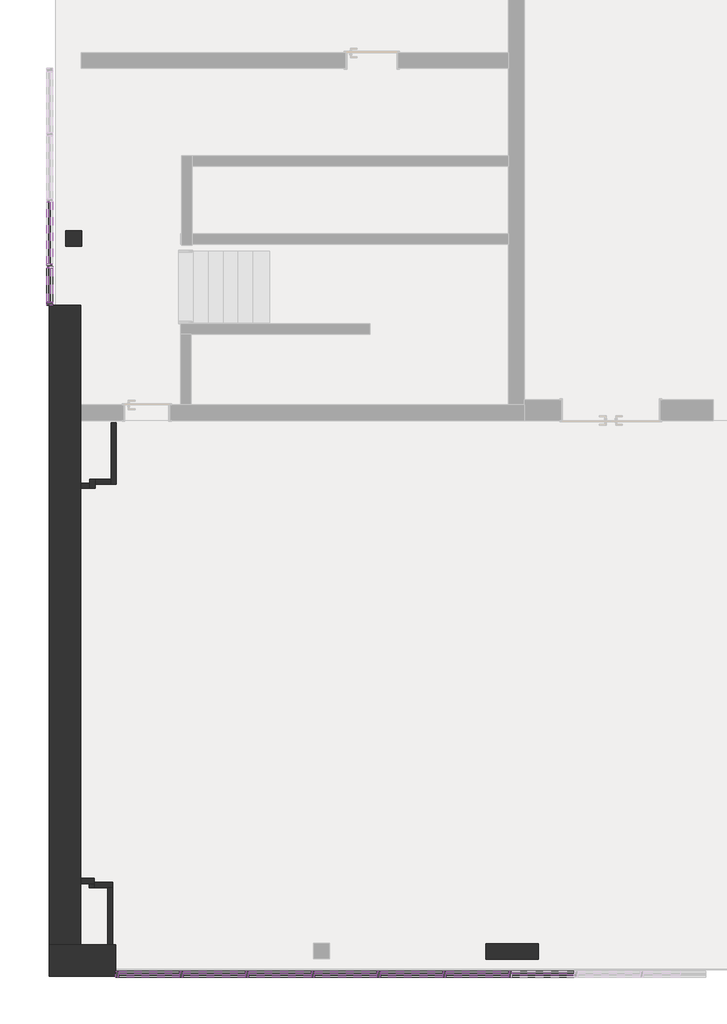
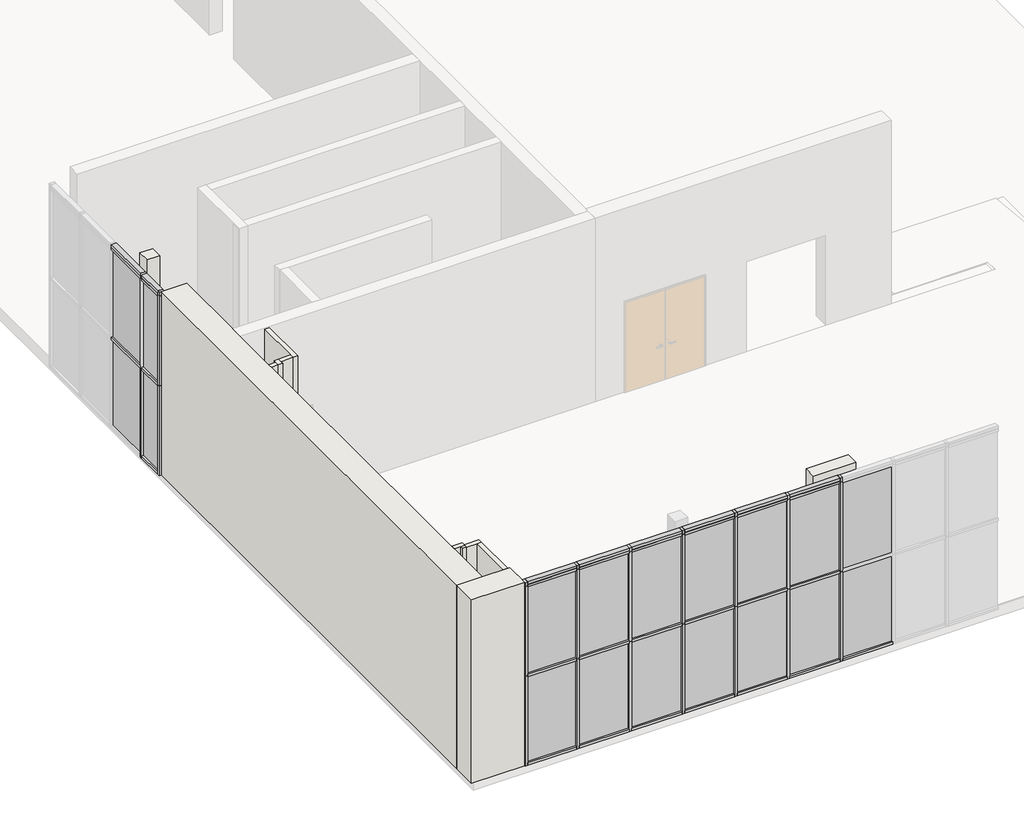
# One storey, part 1 of 5: 57 members, 27 plates, 12 walls.
"""IFC4 building model written with IfcOpenShell, lengths in millimetres."""

import ifcopenshell
import ifcopenshell.guid

model = None  # the IFC model being written
_history = None  # IfcOwnerHistory: only IFC2X3 demands one
_inside = {}  # id of a spatial element -> (the spatial element, [elements in it])
_under = {}  # id of a project, library or spatial element -> (it, [spatial elements below it])
_declared = {}  # id of a project -> (the project, [libraries it declares])
_typed = {}  # id of a type object -> (the type object, [elements of that type])
_made_of = {}  # id of a material, layer set ... -> (it, [elements and type objects made of it])


def new_model(schema):
    """Start an empty IFC model of exactly this schema.

    Asked for "IFC4X3", IfcOpenShell would pick the latest addendum, in which some entities
    have other attributes; the version numbers below select the first issue.
    IFC2X3 requires an IfcOwnerHistory on every rooted entity: one is made here for all.
    """
    global model, _history
    if schema == "IFC4X3":
        model = ifcopenshell.file(schema_version=(4, 3, 0, 0))
    else:
        model = ifcopenshell.file(schema=schema)
    _inside.clear()
    _under.clear()
    _declared.clear()
    _typed.clear()
    _made_of.clear()
    _history = None
    if model.schema == "IFC2X3":
        org = make("IfcOrganization", Name="unknown")
        user = make(
            "IfcPersonAndOrganization",
            ThePerson=make("IfcPerson", FamilyName="unknown"),
            TheOrganization=org,
        )
        app = make(
            "IfcApplication",
            ApplicationDeveloper=org,
            Version="unknown",
            ApplicationFullName="unknown",
            ApplicationIdentifier="unknown",
        )
        _history = make(
            "IfcOwnerHistory",
            OwningUser=user,
            OwningApplication=app,
            ChangeAction="ADDED",
            CreationDate=0,
        )
    return model


def make(cls, **values):
    """One entity of the class cls with the attributes given. An attribute that is None is left unset."""
    return model.create_entity(
        cls, **{name: value for name, value in values.items() if value is not None}
    )


def rooted(cls, **values):
    """An entity with a GlobalId (a new one), such as an element, a storey or a relation."""
    return make(cls, GlobalId=ifcopenshell.guid.new(), OwnerHistory=_history, **values)


def si_unit(unit_type, name, prefix=None):
    """IfcSIUnit, for example si_unit("LENGTHUNIT", "METRE", prefix="MILLI")."""
    return make("IfcSIUnit", UnitType=unit_type, Prefix=prefix, Name=name)


def assignment(units):
    """IfcUnitAssignment: the units of a project."""
    return None if units is None else make("IfcUnitAssignment", Units=units)


def point(xyz):
    """IfcCartesianPoint."""
    return None if xyz is None else make("IfcCartesianPoint", Coordinates=xyz)


def direction(xyz):
    """IfcDirection."""
    return None if xyz is None else make("IfcDirection", DirectionRatios=xyz)


def frame(location, z_axis=None, x_axis=None):
    """IfcAxis2Placement3D, a coordinate frame: its origin and axes. An axis left out is left unset."""
    return make(
        "IfcAxis2Placement3D",
        Location=point(location),
        Axis=direction(z_axis),
        RefDirection=direction(x_axis),
    )


def origin():
    """The frame at (0, 0, 0) with its axes left unset."""
    return frame((0.0, 0.0, 0.0))


def origin_with_axes():
    """The frame at (0, 0, 0) with the z axis (0, 0, 1) and the x axis (1, 0, 0) written out."""
    return frame((0.0, 0.0, 0.0), z_axis=(0.0, 0.0, 1.0), x_axis=(1.0, 0.0, 0.0))


def place(relative_to, where):
    """IfcLocalPlacement: puts the frame where relative to a parent placement (None: the world)."""
    return make(
        "IfcLocalPlacement", PlacementRelTo=relative_to, RelativePlacement=where
    )


def context(
    kind, dimensions, precision=None, world=None, true_north=None, identifier=None
):
    """IfcGeometricRepresentationContext, for example the 3D "Model" context."""
    return make(
        "IfcGeometricRepresentationContext",
        ContextIdentifier=identifier,
        ContextType=kind,
        CoordinateSpaceDimension=dimensions,
        Precision=precision,
        WorldCoordinateSystem=world,
        TrueNorth=true_north,
    )


def project(units=None, contexts=None):
    """IfcProject with its units and contexts."""
    return rooted(
        "IfcProject",
        Name="project",
        RepresentationContexts=contexts,
        UnitsInContext=assignment(units),
    )


def spatial(cls, under=None, at=None, **own):
    """A site, building, storey or space (cls), placed at a placement, below another one or the project."""
    s = rooted(cls, ObjectPlacement=at, **own)
    if under is not None:
        _under.setdefault(under.id(), (under, []))[1].append(s)
    return s


def polyline(points):
    """IfcPolyline through the points."""
    return make("IfcPolyline", Points=[point(p) for p in points])


def outline(outer, holes=None, kind="AREA"):
    """IfcArbitraryClosedProfileDef: a profile drawn as a closed curve; with holes, ...WithVoids."""
    if holes is None:
        return make("IfcArbitraryClosedProfileDef", ProfileType=kind, OuterCurve=outer)
    return make(
        "IfcArbitraryProfileDefWithVoids",
        ProfileType=kind,
        OuterCurve=outer,
        InnerCurves=holes,
    )


def extrude(swept, where, along, depth):
    """IfcExtrudedAreaSolid: the profile swept, set in the frame where, extruded along a direction by depth."""
    return make(
        "IfcExtrudedAreaSolid",
        SweptArea=swept,
        Position=where,
        ExtrudedDirection=direction(along),
        Depth=depth,
    )


def faces_of(points, faces, orient=None, outer=None):
    """IfcFace entities. A face is a list of loops; a loop is a list of indices into points, from 0.

    orient and outer hold one flag for each loop. By default every Orientation is true, the
    first loop of a face is its IfcFaceOuterBound and the others are IfcFaceBound.
    """
    made = []
    for i, loops in enumerate(faces):
        bounds = []
        for j, loop in enumerate(loops):
            is_outer = j == 0 if outer is None else outer[i][j]
            bounds.append(
                make(
                    "IfcFaceOuterBound" if is_outer else "IfcFaceBound",
                    Bound=make("IfcPolyLoop", Polygon=[points[k] for k in loop]),
                    Orientation=True if orient is None else orient[i][j],
                )
            )
        made.append(make("IfcFace", Bounds=bounds))
    return made


def faceted_brep(points, faces, orient=None, outer=None, voids=None):
    """IfcFacetedBrep: a solid bounded by flat faces; with voids (closed shells), ...WithVoids."""
    shared = [point(p) for p in points]
    hull = make("IfcClosedShell", CfsFaces=faces_of(shared, faces, orient, outer))
    if voids is None:
        return make("IfcFacetedBrep", Outer=hull)
    return make(
        "IfcFacetedBrepWithVoids",
        Outer=hull,
        Voids=[
            make(cls, CfsFaces=faces_of(shared, fs, o, b)) for cls, fs, o, b in voids
        ],
    )


def shape(context_of_items, identifier, shape_type, items):
    """IfcShapeRepresentation: the items that make up one representation, for example the "Body"."""
    return make(
        "IfcShapeRepresentation",
        ContextOfItems=context_of_items,
        RepresentationIdentifier=identifier,
        RepresentationType=shape_type,
        Items=items,
    )


def source(mapping_origin, context_of_items, identifier, shape_type, items):
    """IfcRepresentationMap: a shape defined once, which mapped items show again and again."""
    return make(
        "IfcRepresentationMap",
        MappingOrigin=mapping_origin,
        MappedRepresentation=shape(context_of_items, identifier, shape_type, items),
    )


def transform(
    local_origin,
    x_axis=None,
    y_axis=None,
    z_axis=None,
    scale=None,
    scale2=None,
    scale3=None,
    uniform=True,
):
    """IfcCartesianTransformationOperator3D, or its non-uniform kind. x_axis, y_axis, z_axis: its Axis1, 2, 3."""
    if uniform:
        return make(
            "IfcCartesianTransformationOperator3D",
            Axis1=direction(x_axis),
            Axis2=direction(y_axis),
            LocalOrigin=point(local_origin),
            Scale=scale,
            Axis3=direction(z_axis),
        )
    return make(
        "IfcCartesianTransformationOperator3DnonUniform",
        Axis1=direction(x_axis),
        Axis2=direction(y_axis),
        LocalOrigin=point(local_origin),
        Scale=scale,
        Axis3=direction(z_axis),
        Scale2=scale2,
        Scale3=scale3,
    )


def mapped(mapping_source, mapping_target):
    """IfcMappedItem: shows the shape of a source again, moved by a transform."""
    return make(
        "IfcMappedItem", MappingSource=mapping_source, MappingTarget=mapping_target
    )


def made_of(thing, what):
    """Note that an element or type object is made of a material, layer set ...; save() writes the relation."""
    if what is not None:
        _made_of.setdefault(what.id(), (what, []))[1].append(thing)
    return thing


def element(
    cls,
    number,
    at=None,
    inside=None,
    cuts=None,
    type_object=None,
    material=None,
    context=None,
    identifier="Body",
    shape_type=None,
    held_by="IfcProductDefinitionShape",
    body=None,
    shapes=None,
    **own,
):
    """One element of the class cls, such as IfcWall. Its Tag is "e" and its number.

    at: its placement. inside: the storey or other place that contains it. cuts: it is an
    opening in that element (IfcRelVoidsElement). A single representation is given by context,
    identifier, shape_type and body (its items); several are given by shapes. held_by: the class
    of the entity that holds the representations. save() writes the other relations.
    """
    e = rooted(cls, Tag="e%d" % number, ObjectPlacement=at, **own)
    if body is not None:
        shapes = [shape(context, identifier, shape_type, body)]
    if shapes is not None:
        e.Representation = make(held_by, Representations=shapes)
    if inside is not None:
        _inside.setdefault(inside.id(), (inside, []))[1].append(e)
    if cuts is not None:
        rooted(
            "IfcRelVoidsElement", RelatingBuildingElement=cuts, RelatedOpeningElement=e
        )
    if type_object is not None:
        _typed.setdefault(type_object.id(), (type_object, []))[1].append(e)
    return made_of(e, material)


def aggregate(whole, parts):
    """IfcRelAggregates: a whole, such as a stair, and the parts it consists of."""
    return rooted("IfcRelAggregates", RelatingObject=whole, RelatedObjects=parts)


def save(model, path):
    """Write the relations noted so far, then the file.

    IfcRelAggregates (storeys below a building ...), IfcRelContainedInSpatialStructure (elements
    in a storey), IfcRelDefinesByType, IfcRelAssociatesMaterial and IfcRelDeclares: one each for
    every whole, place, type object, material and project.
    """
    for whole, parts in _under.values():
        aggregate(whole, parts)
    for where, things in _inside.values():
        rooted(
            "IfcRelContainedInSpatialStructure",
            RelatedElements=things,
            RelatingStructure=where,
        )
    for kind, things in _typed.values():
        rooted("IfcRelDefinesByType", RelatedObjects=things, RelatingType=kind)
    for what, things in _made_of.values():
        rooted("IfcRelAssociatesMaterial", RelatedObjects=things, RelatingMaterial=what)
    for by, libraries in _declared.values():
        rooted("IfcRelDeclares", RelatingContext=by, RelatedDefinitions=libraries)
    model.write(path)


def pfosten_rechteckig_6_x_12_9384716b(model_context):
    return source(origin(), model_context, "Body", "SweptSolid", [
        extrude(outline(polyline([(0.0, 60.0), (0.0, -60.0), (-60.0, -60.0), (-60.0, 60.0), (0.0, 60.0)])), frame((0.0, 0.0, -1160.0000003), z_axis=(0.0, 0.0, 1.0), x_axis=(1.0, 0.0, 0.0)), (0.0, 0.0, 1.0), 1160.0000003),
    ])


def pfosten_rechteckig_6_x_12_36a2a28f(model_context):
    return source(origin(), model_context, "Body", "SweptSolid", [
        extrude(outline(polyline([(0.0, 60.0), (0.0, -60.0), (-60.0, -60.0), (-60.0, 60.0), (0.0, 60.0)])), frame((0.0, 0.0, -1190.0), z_axis=(0.0, 0.0, 1.0), x_axis=(1.0, 0.0, 0.0)), (0.0, 0.0, 1.0), 1190.0),
    ])


def pfosten_rechteckig_6_x_12_ce3c1f4b(model_context):
    return source(origin(), model_context, "Body", "SweptSolid", [
        extrude(outline(polyline([(30.0, 60.0), (30.0, -60.0), (-30.0, -60.0), (-30.0, 60.0), (30.0, 60.0)])), frame((0.0, 0.0, -1160.0000003), z_axis=(0.0, 0.0, 1.0), x_axis=(1.0, 0.0, 0.0)), (0.0, 0.0, 1.0), 1160.0000003),
    ])


def pfosten_rechteckig_6_x_12_8bb825ca(model_context):
    return source(origin(), model_context, "Body", "SweptSolid", [
        extrude(outline(polyline([(30.0, 60.0), (30.0, -60.0), (-30.0, -60.0), (-30.0, 60.0), (30.0, 60.0)])), frame((0.0, 0.0, -1190.0), z_axis=(0.0, 0.0, 1.0), x_axis=(1.0, 0.0, 0.0)), (0.0, 0.0, 1.0), 1190.0),
    ])


def pfosten_rechteckig_6_x_12_8f909f43(model_context):
    return source(origin(), model_context, "Body", "SweptSolid", [
        extrude(outline(polyline([(30.0, 60.0), (30.0, -60.0), (-30.0, -60.0), (-30.0, 60.0), (30.0, 60.0)])), frame((0.0, 0.0, -2250.0), z_axis=(0.0, 0.0, 1.0), x_axis=(1.0, 0.0, 0.0)), (0.0, 0.0, 1.0), 2250.0),
    ])


def pfosten_rechteckig_6_x_12_b6f87324(model_context):
    return source(origin(), model_context, "Body", "SweptSolid", [
        extrude(outline(polyline([(0.0, 60.0), (0.0, -60.0), (-60.0, -60.0), (-60.0, 60.0), (0.0, 60.0)])), frame((0.0, 0.0, -2250.0), z_axis=(0.0, 0.0, 1.0), x_axis=(1.0, 0.0, 0.0)), (0.0, 0.0, 1.0), 2250.0),
    ])


def pfosten_rechteckig_6_x_12_9d54109d(model_context):
    return source(origin(), model_context, "Body", "SweptSolid", [
        extrude(outline(polyline([(30.0, 60.0), (30.0, -60.0), (-30.0, -60.0), (-30.0, 60.0), (30.0, 60.0)])), frame((0.0, 0.0, -100.0), z_axis=(0.0, 0.0, 1.0), x_axis=(1.0, 0.0, 0.0)), (0.0, 0.0, 1.0), 100.0),
    ])


def pfosten_rechteckig_6_x_12_fc4c2c82(model_context):
    return source(origin(), model_context, "Body", "SweptSolid", [
        extrude(outline(polyline([(0.0, 60.0), (0.0, -60.0), (-60.0, -60.0), (-60.0, 60.0), (0.0, 60.0)])), frame((0.0, 0.0, -100.0), z_axis=(0.0, 0.0, 1.0), x_axis=(1.0, 0.0, 0.0)), (0.0, 0.0, 1.0), 100.0),
    ])


def pfosten_rechteckig_6_x_12_97c23e68(model_context):
    return source(origin(), model_context, "Body", "SweptSolid", [
        extrude(outline(polyline([(0.0, 60.0), (0.0, -60.0), (-60.0, -60.0), (-60.0, 60.0), (0.0, 60.0)])), frame((0.0, 0.0, -660.287322), z_axis=(0.0, 0.0, 1.0), x_axis=(1.0, 0.0, 0.0)), (0.0, 0.0, 1.0), 660.287322),
    ])


def pfosten_rechteckig_6_x_12_e841a96c(model_context):
    return source(origin(), model_context, "Body", "SweptSolid", [
        extrude(outline(polyline([(30.0, 60.0), (30.0, -60.0), (-30.0, -60.0), (-30.0, 60.0), (30.0, 60.0)])), frame((0.0, 0.0, -660.287322), z_axis=(0.0, 0.0, 1.0), x_axis=(1.0, 0.0, 0.0)), (0.0, 0.0, 1.0), 660.287322),
    ])


def systemelement_verglasung_ac3f6550(model_context):
    return source(origin(), model_context, "Body", "SweptSolid", [
        extrude(outline(polyline([(580.0000002, -15.0), (-580.0000002, -15.0), (-580.0000002, 15.0), (580.0000002, 15.0), (580.0000002, -15.0)])), origin_with_axes(), (0.0, 0.0, 1.0), 2160.0),
    ])


def systemelement_verglasung_d38c8d2b(model_context):
    return source(origin(), model_context, "Body", "SweptSolid", [
        extrude(outline(polyline([(595.0, -15.0), (-595.0, -15.0), (-595.0, 15.0), (595.0, 15.0), (595.0, -15.0)])), origin_with_axes(), (0.0, 0.0, 1.0), 2160.0),
    ])


def systemelement_verglasung_7f313b09(model_context):
    return source(origin(), model_context, "Body", "SweptSolid", [
        extrude(outline(polyline([(580.0000002, -15.0), (-580.0000002, -15.0), (-580.0000002, 15.0), (580.0000002, 15.0), (580.0000002, -15.0)])), origin_with_axes(), (0.0, 0.0, 1.0), 2190.0),
    ])


def systemelement_verglasung_4115e844(model_context):
    return source(origin(), model_context, "Body", "SweptSolid", [
        extrude(outline(polyline([(595.0, -15.0), (-595.0, -15.0), (-595.0, 15.0), (595.0, 15.0), (595.0, -15.0)])), origin_with_axes(), (0.0, 0.0, 1.0), 2190.0),
    ])


def systemelement_verglasung_1bc3a817(model_context):
    return source(origin(), model_context, "Body", "SweptSolid", [
        extrude(outline(polyline([(580.0000002, -15.0), (-580.0000002, -15.0), (-580.0000002, 15.0), (580.0000002, 15.0), (580.0000002, -15.0)])), origin_with_axes(), (0.0, 0.0, 1.0), 10.0),
    ])


def systemelement_verglasung_dd9543b1(model_context):
    return source(origin(), model_context, "Body", "SweptSolid", [
        extrude(outline(polyline([(595.0, -15.0), (-595.0, -15.0), (-595.0, 15.0), (595.0, 15.0), (595.0, -15.0)])), origin_with_axes(), (0.0, 0.0, 1.0), 10.0),
    ])


def systemelement_verglasung_92099b16(model_context):
    return source(origin(), model_context, "Body", "SweptSolid", [
        extrude(outline(polyline([(330.143661, -15.0), (-330.143661, -15.0), (-330.143661, 15.0), (330.143661, 15.0), (330.143661, -15.0)])), origin_with_axes(), (0.0, 0.0, 1.0), 2160.0),
    ])


def systemelement_verglasung_ac39db88(model_context):
    return source(origin(), model_context, "Body", "SweptSolid", [
        extrude(outline(polyline([(330.143661, -15.0), (-330.143661, -15.0), (-330.143661, 15.0), (330.143661, 15.0), (330.143661, -15.0)])), origin_with_axes(), (0.0, 0.0, 1.0), 2190.0),
    ])


def systemelement_verglasung_0eadd769(model_context):
    return source(origin(), model_context, "Body", "SweptSolid", [
        extrude(outline(polyline([(330.143661, -15.0), (-330.143661, -15.0), (-330.143661, 15.0), (330.143661, 15.0), (330.143661, -15.0)])), origin_with_axes(), (0.0, 0.0, 1.0), 10.0),
    ])


model = new_model("IFC4")

# Units and contexts
model_context = context("Model", 3, world=origin())
ifc_project = project(units=[si_unit("LENGTHUNIT", "METRE", prefix="MILLI")], contexts=[model_context])

# Site, building, storey
site = spatial("IfcSite", under=ifc_project)
building = spatial("IfcBuilding", under=site)
storey = spatial("IfcBuildingStorey", under=building, Name="EFH", Elevation=-1570.0)

# Members
placement = place(None, origin())
pfosten_rechteckig_6_x_12_shape = pfosten_rechteckig_6_x_12_9384716b(model_context)
element("IfcMember", 1, ObjectType="Pfosten rechteckig : 6 x 12", at=placement, inside=storey, context=model_context, shape_type="MappedRepresentation", body=[
    mapped(pfosten_rechteckig_6_x_12_shape, transform((-8503.177684, -15149.0347147, -1570.0), x_axis=(0.0, 0.0, -1.0), y_axis=(0.0, -1.0, 0.0), z_axis=(-1.0, 0.0, 0.0))),
])
element("IfcMember", 2, ObjectType="Pfosten rechteckig : 6 x 12", at=placement, inside=storey, context=model_context, shape_type="MappedRepresentation", body=[
    mapped(pfosten_rechteckig_6_x_12_shape, transform((-7343.1776837, -15149.0347147, 3030.0), x_axis=(0.0, 0.0, 1.0), y_axis=(0.0, -1.0, 0.0), z_axis=(1.0, 0.0, 0.0))),
])
pfosten_rechteckig_6_x_12_2_shape = pfosten_rechteckig_6_x_12_36a2a28f(model_context)
element("IfcMember", 3, ObjectType="Pfosten rechteckig : 6 x 12", at=placement, inside=storey, context=model_context, shape_type="MappedRepresentation", body=[
    mapped(pfosten_rechteckig_6_x_12_2_shape, transform((-6093.1776837, -15149.0347147, 3030.0), x_axis=(0.0, 0.0, 1.0), y_axis=(0.0, -1.0, 0.0), z_axis=(1.0, 0.0, 0.0))),
])
element("IfcMember", 4, ObjectType="Pfosten rechteckig : 6 x 12", at=placement, inside=storey, context=model_context, shape_type="MappedRepresentation", body=[
    mapped(pfosten_rechteckig_6_x_12_2_shape, transform((-4843.1776837, -15149.0347147, 3030.0), x_axis=(0.0, 0.0, 1.0), y_axis=(0.0, -1.0, 0.0), z_axis=(1.0, 0.0, 0.0))),
])
element("IfcMember", 5, ObjectType="Pfosten rechteckig : 6 x 12", at=placement, inside=storey, context=model_context, shape_type="MappedRepresentation", body=[
    mapped(pfosten_rechteckig_6_x_12_2_shape, transform((-3593.1776837, -15149.0347147, 3030.0), x_axis=(0.0, 0.0, 1.0), y_axis=(0.0, -1.0, 0.0), z_axis=(1.0, 0.0, 0.0))),
])
element("IfcMember", 6, ObjectType="Pfosten rechteckig : 6 x 12", at=placement, inside=storey, context=model_context, shape_type="MappedRepresentation", body=[
    mapped(pfosten_rechteckig_6_x_12_2_shape, transform((-2343.1776837, -15149.0347147, 3030.0), x_axis=(0.0, 0.0, 1.0), y_axis=(0.0, -1.0, 0.0), z_axis=(1.0, 0.0, 0.0))),
])
element("IfcMember", 7, ObjectType="Pfosten rechteckig : 6 x 12", at=placement, inside=storey, context=model_context, shape_type="MappedRepresentation", body=[
    mapped(pfosten_rechteckig_6_x_12_2_shape, transform((-1093.1776837, -15149.0347147, 3030.0), x_axis=(0.0, 0.0, 1.0), y_axis=(0.0, -1.0, 0.0), z_axis=(1.0, 0.0, 0.0))),
])
element("IfcMember", 8, ObjectType="Pfosten rechteckig : 6 x 12", at=placement, inside=storey, context=model_context, shape_type="MappedRepresentation", body=[
    mapped(pfosten_rechteckig_6_x_12_2_shape, transform((-9817.3070453, -1665.6888999, 3030.0), x_axis=(0.0, 0.0, 1.0), y_axis=(-1.0, 0.0, 0.0), z_axis=(0.0, -1.0, 0.0))),
])
element("IfcMember", 9, ObjectType="Pfosten rechteckig : 6 x 12", at=placement, inside=storey, context=model_context, shape_type="MappedRepresentation", body=[
    mapped(pfosten_rechteckig_6_x_12_2_shape, transform((-7283.1776837, -15149.0347147, -1570.0), x_axis=(0.0, 0.0, -1.0), y_axis=(0.0, -1.0, 0.0), z_axis=(-1.0, 0.0, 0.0))),
])
element("IfcMember", 10, ObjectType="Pfosten rechteckig : 6 x 12", at=placement, inside=storey, context=model_context, shape_type="MappedRepresentation", body=[
    mapped(pfosten_rechteckig_6_x_12_2_shape, transform((-6033.1776837, -15149.0347147, -1570.0), x_axis=(0.0, 0.0, -1.0), y_axis=(0.0, -1.0, 0.0), z_axis=(-1.0, 0.0, 0.0))),
])
element("IfcMember", 11, ObjectType="Pfosten rechteckig : 6 x 12", at=placement, inside=storey, context=model_context, shape_type="MappedRepresentation", body=[
    mapped(pfosten_rechteckig_6_x_12_2_shape, transform((-4783.1776837, -15149.0347147, -1570.0), x_axis=(0.0, 0.0, -1.0), y_axis=(0.0, -1.0, 0.0), z_axis=(-1.0, 0.0, 0.0))),
])
element("IfcMember", 12, ObjectType="Pfosten rechteckig : 6 x 12", at=placement, inside=storey, context=model_context, shape_type="MappedRepresentation", body=[
    mapped(pfosten_rechteckig_6_x_12_2_shape, transform((-3533.1776837, -15149.0347147, -1570.0), x_axis=(0.0, 0.0, -1.0), y_axis=(0.0, -1.0, 0.0), z_axis=(-1.0, 0.0, 0.0))),
])
element("IfcMember", 13, ObjectType="Pfosten rechteckig : 6 x 12", at=placement, inside=storey, context=model_context, shape_type="MappedRepresentation", body=[
    mapped(pfosten_rechteckig_6_x_12_2_shape, transform((-2283.1776837, -15149.0347147, -1570.0), x_axis=(0.0, 0.0, -1.0), y_axis=(0.0, -1.0, 0.0), z_axis=(-1.0, 0.0, 0.0))),
])
element("IfcMember", 14, ObjectType="Pfosten rechteckig : 6 x 12", at=placement, inside=storey, context=model_context, shape_type="MappedRepresentation", body=[
    mapped(pfosten_rechteckig_6_x_12_2_shape, transform((-1033.1776837, -15149.0347147, -1570.0), x_axis=(0.0, 0.0, -1.0), y_axis=(0.0, -1.0, 0.0), z_axis=(-1.0, 0.0, 0.0))),
])
pfosten_rechteckig_6_x_12_3_shape = pfosten_rechteckig_6_x_12_ce3c1f4b(model_context)
element("IfcMember", 15, ObjectType="Pfosten rechteckig : 6 x 12", at=placement, inside=storey, context=model_context, shape_type="MappedRepresentation", body=[
    mapped(pfosten_rechteckig_6_x_12_3_shape, transform((-7343.1776837, -15149.0347147, 680.0), x_axis=(0.0, 0.0, 1.0), y_axis=(0.0, -1.0, 0.0), z_axis=(1.0, 0.0, 0.0))),
])
element("IfcMember", 16, ObjectType="Pfosten rechteckig : 6 x 12", at=placement, inside=storey, context=model_context, shape_type="MappedRepresentation", body=[
    mapped(pfosten_rechteckig_6_x_12_3_shape, transform((-7343.1776837, -15149.0347147, 2930.0), x_axis=(0.0, 0.0, 1.0), y_axis=(0.0, -1.0, 0.0), z_axis=(1.0, 0.0, 0.0))),
])
pfosten_rechteckig_6_x_12_4_shape = pfosten_rechteckig_6_x_12_8bb825ca(model_context)
element("IfcMember", 17, ObjectType="Pfosten rechteckig : 6 x 12", at=placement, inside=storey, context=model_context, shape_type="MappedRepresentation", body=[
    mapped(pfosten_rechteckig_6_x_12_4_shape, transform((-6093.1776837, -15149.0347147, 680.0), x_axis=(0.0, 0.0, 1.0), y_axis=(0.0, -1.0, 0.0), z_axis=(1.0, 0.0, 0.0))),
])
element("IfcMember", 18, ObjectType="Pfosten rechteckig : 6 x 12", at=placement, inside=storey, context=model_context, shape_type="MappedRepresentation", body=[
    mapped(pfosten_rechteckig_6_x_12_4_shape, transform((-4843.1776837, -15149.0347147, 680.0), x_axis=(0.0, 0.0, 1.0), y_axis=(0.0, -1.0, 0.0), z_axis=(1.0, 0.0, 0.0))),
])
element("IfcMember", 19, ObjectType="Pfosten rechteckig : 6 x 12", at=placement, inside=storey, context=model_context, shape_type="MappedRepresentation", body=[
    mapped(pfosten_rechteckig_6_x_12_4_shape, transform((-3593.1776837, -15149.0347147, 680.0), x_axis=(0.0, 0.0, 1.0), y_axis=(0.0, -1.0, 0.0), z_axis=(1.0, 0.0, 0.0))),
])
element("IfcMember", 20, ObjectType="Pfosten rechteckig : 6 x 12", at=placement, inside=storey, context=model_context, shape_type="MappedRepresentation", body=[
    mapped(pfosten_rechteckig_6_x_12_4_shape, transform((-2343.1776837, -15149.0347147, 680.0), x_axis=(0.0, 0.0, 1.0), y_axis=(0.0, -1.0, 0.0), z_axis=(1.0, 0.0, 0.0))),
])
element("IfcMember", 21, ObjectType="Pfosten rechteckig : 6 x 12", at=placement, inside=storey, context=model_context, shape_type="MappedRepresentation", body=[
    mapped(pfosten_rechteckig_6_x_12_4_shape, transform((-1093.1776837, -15149.0347147, 680.0), x_axis=(0.0, 0.0, 1.0), y_axis=(0.0, -1.0, 0.0), z_axis=(1.0, 0.0, 0.0))),
])
element("IfcMember", 22, ObjectType="Pfosten rechteckig : 6 x 12", at=placement, inside=storey, context=model_context, shape_type="MappedRepresentation", body=[
    mapped(pfosten_rechteckig_6_x_12_4_shape, transform((-6093.1776837, -15149.0347147, 2930.0), x_axis=(0.0, 0.0, 1.0), y_axis=(0.0, -1.0, 0.0), z_axis=(1.0, 0.0, 0.0))),
])
element("IfcMember", 23, ObjectType="Pfosten rechteckig : 6 x 12", at=placement, inside=storey, context=model_context, shape_type="MappedRepresentation", body=[
    mapped(pfosten_rechteckig_6_x_12_4_shape, transform((-4843.1776837, -15149.0347147, 2930.0), x_axis=(0.0, 0.0, 1.0), y_axis=(0.0, -1.0, 0.0), z_axis=(1.0, 0.0, 0.0))),
])
element("IfcMember", 24, ObjectType="Pfosten rechteckig : 6 x 12", at=placement, inside=storey, context=model_context, shape_type="MappedRepresentation", body=[
    mapped(pfosten_rechteckig_6_x_12_4_shape, transform((-3593.1776837, -15149.0347147, 2930.0), x_axis=(0.0, 0.0, 1.0), y_axis=(0.0, -1.0, 0.0), z_axis=(1.0, 0.0, 0.0))),
])
element("IfcMember", 25, ObjectType="Pfosten rechteckig : 6 x 12", at=placement, inside=storey, context=model_context, shape_type="MappedRepresentation", body=[
    mapped(pfosten_rechteckig_6_x_12_4_shape, transform((-2343.1776837, -15149.0347147, 2930.0), x_axis=(0.0, 0.0, 1.0), y_axis=(0.0, -1.0, 0.0), z_axis=(1.0, 0.0, 0.0))),
])
element("IfcMember", 26, ObjectType="Pfosten rechteckig : 6 x 12", at=placement, inside=storey, context=model_context, shape_type="MappedRepresentation", body=[
    mapped(pfosten_rechteckig_6_x_12_4_shape, transform((-1093.1776837, -15149.0347147, 2930.0), x_axis=(0.0, 0.0, 1.0), y_axis=(0.0, -1.0, 0.0), z_axis=(1.0, 0.0, 0.0))),
])
element("IfcMember", 27, ObjectType="Pfosten rechteckig : 6 x 12", at=placement, inside=storey, context=model_context, shape_type="MappedRepresentation", body=[
    mapped(pfosten_rechteckig_6_x_12_4_shape, transform((-9817.3070453, -1665.6888999, 680.0), x_axis=(0.0, 0.0, 1.0), y_axis=(-1.0, 0.0, 0.0), z_axis=(0.0, -1.0, 0.0))),
])
element("IfcMember", 28, ObjectType="Pfosten rechteckig : 6 x 12", at=placement, inside=storey, context=model_context, shape_type="MappedRepresentation", body=[
    mapped(pfosten_rechteckig_6_x_12_4_shape, transform((-9817.3070453, -1665.6888999, 2930.0), x_axis=(0.0, 0.0, 1.0), y_axis=(-1.0, 0.0, 0.0), z_axis=(0.0, -1.0, 0.0))),
])
pfosten_rechteckig_6_x_12_5_shape = pfosten_rechteckig_6_x_12_8f909f43(model_context)
element("IfcMember", 29, ObjectType="Pfosten rechteckig : 6 x 12", at=placement, inside=storey, context=model_context, shape_type="MappedRepresentation", body=[
    mapped(pfosten_rechteckig_6_x_12_5_shape, transform((-7313.1776837, -15149.0347147, -1570.0), x_axis=(1.0, 0.0, 0.0), y_axis=(0.0, -1.0, 0.0), z_axis=(0.0, 0.0, -1.0))),
])
element("IfcMember", 30, ObjectType="Pfosten rechteckig : 6 x 12", at=placement, inside=storey, context=model_context, shape_type="MappedRepresentation", body=[
    mapped(pfosten_rechteckig_6_x_12_5_shape, transform((-6063.1776837, -15149.0347147, -1570.0), x_axis=(1.0, 0.0, 0.0), y_axis=(0.0, -1.0, 0.0), z_axis=(0.0, 0.0, -1.0))),
])
element("IfcMember", 31, ObjectType="Pfosten rechteckig : 6 x 12", at=placement, inside=storey, context=model_context, shape_type="MappedRepresentation", body=[
    mapped(pfosten_rechteckig_6_x_12_5_shape, transform((-4813.1776837, -15149.0347147, -1570.0), x_axis=(1.0, 0.0, 0.0), y_axis=(0.0, -1.0, 0.0), z_axis=(0.0, 0.0, -1.0))),
])
element("IfcMember", 32, ObjectType="Pfosten rechteckig : 6 x 12", at=placement, inside=storey, context=model_context, shape_type="MappedRepresentation", body=[
    mapped(pfosten_rechteckig_6_x_12_5_shape, transform((-3563.1776837, -15149.0347147, -1570.0), x_axis=(1.0, 0.0, 0.0), y_axis=(0.0, -1.0, 0.0), z_axis=(0.0, 0.0, -1.0))),
])
element("IfcMember", 33, ObjectType="Pfosten rechteckig : 6 x 12", at=placement, inside=storey, context=model_context, shape_type="MappedRepresentation", body=[
    mapped(pfosten_rechteckig_6_x_12_5_shape, transform((-2313.1776837, -15149.0347147, -1570.0), x_axis=(1.0, 0.0, 0.0), y_axis=(0.0, -1.0, 0.0), z_axis=(0.0, 0.0, -1.0))),
])
element("IfcMember", 34, ObjectType="Pfosten rechteckig : 6 x 12", at=placement, inside=storey, context=model_context, shape_type="MappedRepresentation", body=[
    mapped(pfosten_rechteckig_6_x_12_5_shape, transform((-1063.1776837, -15149.0347147, -1570.0), x_axis=(1.0, 0.0, 0.0), y_axis=(0.0, -1.0, 0.0), z_axis=(0.0, 0.0, -1.0))),
])
element("IfcMember", 35, ObjectType="Pfosten rechteckig : 6 x 12", at=placement, inside=storey, context=model_context, shape_type="MappedRepresentation", body=[
    mapped(pfosten_rechteckig_6_x_12_5_shape, transform((-9817.3070453, -1695.6888999, -1570.0), x_axis=(0.0, -1.0, 0.0), y_axis=(-1.0, 0.0, 0.0), z_axis=(0.0, 0.0, -1.0))),
])
element("IfcMember", 36, ObjectType="Pfosten rechteckig : 6 x 12", at=placement, inside=storey, context=model_context, shape_type="MappedRepresentation", body=[
    mapped(pfosten_rechteckig_6_x_12_5_shape, transform((-7313.1776837, -15149.0347147, 680.0), x_axis=(1.0, 0.0, 0.0), y_axis=(0.0, -1.0, 0.0), z_axis=(0.0, 0.0, -1.0))),
])
element("IfcMember", 37, ObjectType="Pfosten rechteckig : 6 x 12", at=placement, inside=storey, context=model_context, shape_type="MappedRepresentation", body=[
    mapped(pfosten_rechteckig_6_x_12_5_shape, transform((-6063.1776837, -15149.0347147, 680.0), x_axis=(1.0, 0.0, 0.0), y_axis=(0.0, -1.0, 0.0), z_axis=(0.0, 0.0, -1.0))),
])
element("IfcMember", 38, ObjectType="Pfosten rechteckig : 6 x 12", at=placement, inside=storey, context=model_context, shape_type="MappedRepresentation", body=[
    mapped(pfosten_rechteckig_6_x_12_5_shape, transform((-4813.1776837, -15149.0347147, 680.0), x_axis=(1.0, 0.0, 0.0), y_axis=(0.0, -1.0, 0.0), z_axis=(0.0, 0.0, -1.0))),
])
element("IfcMember", 39, ObjectType="Pfosten rechteckig : 6 x 12", at=placement, inside=storey, context=model_context, shape_type="MappedRepresentation", body=[
    mapped(pfosten_rechteckig_6_x_12_5_shape, transform((-3563.1776837, -15149.0347147, 680.0), x_axis=(1.0, 0.0, 0.0), y_axis=(0.0, -1.0, 0.0), z_axis=(0.0, 0.0, -1.0))),
])
element("IfcMember", 40, ObjectType="Pfosten rechteckig : 6 x 12", at=placement, inside=storey, context=model_context, shape_type="MappedRepresentation", body=[
    mapped(pfosten_rechteckig_6_x_12_5_shape, transform((-2313.1776837, -15149.0347147, 680.0), x_axis=(1.0, 0.0, 0.0), y_axis=(0.0, -1.0, 0.0), z_axis=(0.0, 0.0, -1.0))),
])
element("IfcMember", 41, ObjectType="Pfosten rechteckig : 6 x 12", at=placement, inside=storey, context=model_context, shape_type="MappedRepresentation", body=[
    mapped(pfosten_rechteckig_6_x_12_5_shape, transform((-1063.1776837, -15149.0347147, 680.0), x_axis=(1.0, 0.0, 0.0), y_axis=(0.0, -1.0, 0.0), z_axis=(0.0, 0.0, -1.0))),
])
pfosten_rechteckig_6_x_12_6_shape = pfosten_rechteckig_6_x_12_b6f87324(model_context)
element("IfcMember", 42, ObjectType="Pfosten rechteckig : 6 x 12", at=placement, inside=storey, context=model_context, shape_type="MappedRepresentation", body=[
    mapped(pfosten_rechteckig_6_x_12_6_shape, transform((-9817.3070453, -2445.9762219, -1570.0), x_axis=(0.0, -1.0, 0.0), y_axis=(-1.0, 0.0, 0.0), z_axis=(0.0, 0.0, -1.0))),
])
element("IfcMember", 43, ObjectType="Pfosten rechteckig : 6 x 12", at=placement, inside=storey, context=model_context, shape_type="MappedRepresentation", body=[
    mapped(pfosten_rechteckig_6_x_12_6_shape, transform((-9817.3070453, -2445.9762219, 680.0), x_axis=(0.0, -1.0, 0.0), y_axis=(-1.0, 0.0, 0.0), z_axis=(0.0, 0.0, -1.0))),
])
element("IfcMember", 44, ObjectType="Pfosten rechteckig : 6 x 12", at=placement, inside=storey, context=model_context, shape_type="MappedRepresentation", body=[
    mapped(pfosten_rechteckig_6_x_12_6_shape, transform((-8563.177684, -15149.0347147, 680.0), x_axis=(-1.0, 0.0, 0.0), y_axis=(0.0, -1.0, 0.0), z_axis=(0.0, 0.0, 1.0))),
])
element("IfcMember", 45, ObjectType="Pfosten rechteckig : 6 x 12", at=placement, inside=storey, context=model_context, shape_type="MappedRepresentation", body=[
    mapped(pfosten_rechteckig_6_x_12_6_shape, transform((-8563.177684, -15149.0347147, 2930.0), x_axis=(-1.0, 0.0, 0.0), y_axis=(0.0, -1.0, 0.0), z_axis=(0.0, 0.0, 1.0))),
])
pfosten_rechteckig_6_x_12_7_shape = pfosten_rechteckig_6_x_12_9d54109d(model_context)
element("IfcMember", 46, ObjectType="Pfosten rechteckig : 6 x 12", at=placement, inside=storey, context=model_context, shape_type="MappedRepresentation", body=[
    mapped(pfosten_rechteckig_6_x_12_7_shape, transform((-7313.1776837, -15149.0347147, 2930.0), x_axis=(1.0, 0.0, 0.0), y_axis=(0.0, -1.0, 0.0), z_axis=(0.0, 0.0, -1.0))),
])
element("IfcMember", 47, ObjectType="Pfosten rechteckig : 6 x 12", at=placement, inside=storey, context=model_context, shape_type="MappedRepresentation", body=[
    mapped(pfosten_rechteckig_6_x_12_7_shape, transform((-6063.1776837, -15149.0347147, 2930.0), x_axis=(1.0, 0.0, 0.0), y_axis=(0.0, -1.0, 0.0), z_axis=(0.0, 0.0, -1.0))),
])
element("IfcMember", 48, ObjectType="Pfosten rechteckig : 6 x 12", at=placement, inside=storey, context=model_context, shape_type="MappedRepresentation", body=[
    mapped(pfosten_rechteckig_6_x_12_7_shape, transform((-4813.1776837, -15149.0347147, 2930.0), x_axis=(1.0, 0.0, 0.0), y_axis=(0.0, -1.0, 0.0), z_axis=(0.0, 0.0, -1.0))),
])
element("IfcMember", 49, ObjectType="Pfosten rechteckig : 6 x 12", at=placement, inside=storey, context=model_context, shape_type="MappedRepresentation", body=[
    mapped(pfosten_rechteckig_6_x_12_7_shape, transform((-3563.1776837, -15149.0347147, 2930.0), x_axis=(1.0, 0.0, 0.0), y_axis=(0.0, -1.0, 0.0), z_axis=(0.0, 0.0, -1.0))),
])
element("IfcMember", 50, ObjectType="Pfosten rechteckig : 6 x 12", at=placement, inside=storey, context=model_context, shape_type="MappedRepresentation", body=[
    mapped(pfosten_rechteckig_6_x_12_7_shape, transform((-2313.1776837, -15149.0347147, 2930.0), x_axis=(1.0, 0.0, 0.0), y_axis=(0.0, -1.0, 0.0), z_axis=(0.0, 0.0, -1.0))),
])
element("IfcMember", 51, ObjectType="Pfosten rechteckig : 6 x 12", at=placement, inside=storey, context=model_context, shape_type="MappedRepresentation", body=[
    mapped(pfosten_rechteckig_6_x_12_7_shape, transform((-1063.1776837, -15149.0347147, 2930.0), x_axis=(1.0, 0.0, 0.0), y_axis=(0.0, -1.0, 0.0), z_axis=(0.0, 0.0, -1.0))),
])
pfosten_rechteckig_6_x_12_8_shape = pfosten_rechteckig_6_x_12_fc4c2c82(model_context)
element("IfcMember", 52, ObjectType="Pfosten rechteckig : 6 x 12", at=placement, inside=storey, context=model_context, shape_type="MappedRepresentation", body=[
    mapped(pfosten_rechteckig_6_x_12_8_shape, transform((-8563.177684, -15149.0347147, 3030.0), x_axis=(-1.0, 0.0, 0.0), y_axis=(0.0, -1.0, 0.0), z_axis=(0.0, 0.0, 1.0))),
])
element("IfcMember", 53, ObjectType="Pfosten rechteckig : 6 x 12", at=placement, inside=storey, context=model_context, shape_type="MappedRepresentation", body=[
    mapped(pfosten_rechteckig_6_x_12_8_shape, transform((-9817.3070453, -2445.9762219, 2930.0), x_axis=(0.0, -1.0, 0.0), y_axis=(-1.0, 0.0, 0.0), z_axis=(0.0, 0.0, -1.0))),
])
pfosten_rechteckig_6_x_12_9_shape = pfosten_rechteckig_6_x_12_97c23e68(model_context)
element("IfcMember", 54, ObjectType="Pfosten rechteckig : 6 x 12", at=placement, inside=storey, context=model_context, shape_type="MappedRepresentation", body=[
    mapped(pfosten_rechteckig_6_x_12_9_shape, transform((-9817.3070453, -2385.9762219, 3030.0), x_axis=(0.0, 0.0, 1.0), y_axis=(-1.0, 0.0, 0.0), z_axis=(0.0, -1.0, 0.0))),
])
element("IfcMember", 55, ObjectType="Pfosten rechteckig : 6 x 12", at=placement, inside=storey, context=model_context, shape_type="MappedRepresentation", body=[
    mapped(pfosten_rechteckig_6_x_12_9_shape, transform((-9817.3070453, -1725.6888999, -1570.0), x_axis=(0.0, 0.0, -1.0), y_axis=(-1.0, 0.0, 0.0), z_axis=(0.0, 1.0, 0.0))),
])
pfosten_rechteckig_6_x_12_10_shape = pfosten_rechteckig_6_x_12_e841a96c(model_context)
element("IfcMember", 56, ObjectType="Pfosten rechteckig : 6 x 12", at=placement, inside=storey, context=model_context, shape_type="MappedRepresentation", body=[
    mapped(pfosten_rechteckig_6_x_12_10_shape, transform((-9817.3070453, -2385.9762219, 680.0), x_axis=(0.0, 0.0, 1.0), y_axis=(-1.0, 0.0, 0.0), z_axis=(0.0, -1.0, 0.0))),
])
element("IfcMember", 57, ObjectType="Pfosten rechteckig : 6 x 12", at=placement, inside=storey, context=model_context, shape_type="MappedRepresentation", body=[
    mapped(pfosten_rechteckig_6_x_12_10_shape, transform((-9817.3070453, -2385.9762219, 2930.0), x_axis=(0.0, 0.0, 1.0), y_axis=(-1.0, 0.0, 0.0), z_axis=(0.0, -1.0, 0.0))),
])

# Plates
systemelement_verglasung_shape = systemelement_verglasung_ac3f6550(model_context)
element("IfcPlate", 58, ObjectType="Systemelement : Verglasung", at=placement, inside=storey, context=model_context, shape_type="MappedRepresentation", body=[
    mapped(systemelement_verglasung_shape, transform((-7923.1776838, -15149.0347147, -1510.0), x_axis=(1.0, 0.0, 0.0), y_axis=(0.0, 1.0, 0.0), z_axis=(0.0, 0.0, 1.0))),
])
systemelement_verglasung_2_shape = systemelement_verglasung_d38c8d2b(model_context)
element("IfcPlate", 59, ObjectType="Systemelement : Verglasung", at=placement, inside=storey, context=model_context, shape_type="MappedRepresentation", body=[
    mapped(systemelement_verglasung_2_shape, transform((-6688.1776837, -15149.0347147, -1510.0), x_axis=(1.0, 0.0, 0.0), y_axis=(0.0, 1.0, 0.0), z_axis=(0.0, 0.0, 1.0))),
])
element("IfcPlate", 60, ObjectType="Systemelement : Verglasung", at=placement, inside=storey, context=model_context, shape_type="MappedRepresentation", body=[
    mapped(systemelement_verglasung_2_shape, transform((-5438.1776837, -15149.0347147, -1510.0), x_axis=(1.0, 0.0, 0.0), y_axis=(0.0, 1.0, 0.0), z_axis=(0.0, 0.0, 1.0))),
])
element("IfcPlate", 61, ObjectType="Systemelement : Verglasung", at=placement, inside=storey, context=model_context, shape_type="MappedRepresentation", body=[
    mapped(systemelement_verglasung_2_shape, transform((-4188.1776837, -15149.0347147, -1510.0), x_axis=(1.0, 0.0, 0.0), y_axis=(0.0, 1.0, 0.0), z_axis=(0.0, 0.0, 1.0))),
])
element("IfcPlate", 62, ObjectType="Systemelement : Verglasung", at=placement, inside=storey, context=model_context, shape_type="MappedRepresentation", body=[
    mapped(systemelement_verglasung_2_shape, transform((-2938.1776837, -15149.0347147, -1510.0), x_axis=(1.0, 0.0, 0.0), y_axis=(0.0, 1.0, 0.0), z_axis=(0.0, 0.0, 1.0))),
])
element("IfcPlate", 63, ObjectType="Systemelement : Verglasung", at=placement, inside=storey, context=model_context, shape_type="MappedRepresentation", body=[
    mapped(systemelement_verglasung_2_shape, transform((-1688.1776837, -15149.0347147, -1510.0), x_axis=(1.0, 0.0, 0.0), y_axis=(0.0, 1.0, 0.0), z_axis=(0.0, 0.0, 1.0))),
])
element("IfcPlate", 64, ObjectType="Systemelement : Verglasung", at=placement, inside=storey, context=model_context, shape_type="MappedRepresentation", body=[
    mapped(systemelement_verglasung_2_shape, transform((-438.1776837, -15149.0347147, -1510.0), x_axis=(1.0, 0.0, 0.0), y_axis=(0.0, 1.0, 0.0), z_axis=(0.0, 0.0, 1.0))),
])
element("IfcPlate", 65, ObjectType="Systemelement : Verglasung", at=placement, inside=storey, context=model_context, shape_type="MappedRepresentation", body=[
    mapped(systemelement_verglasung_2_shape, transform((-9817.3070453, -1070.6888999, -1510.0), x_axis=(0.0, -1.0, 0.0), y_axis=(1.0, 0.0, 0.0), z_axis=(0.0, 0.0, 1.0))),
])
systemelement_verglasung_3_shape = systemelement_verglasung_7f313b09(model_context)
element("IfcPlate", 66, ObjectType="Systemelement : Verglasung", at=placement, inside=storey, context=model_context, shape_type="MappedRepresentation", body=[
    mapped(systemelement_verglasung_3_shape, transform((-7923.1776838, -15149.0347147, 710.0), x_axis=(1.0, 0.0, 0.0), y_axis=(0.0, 1.0, 0.0), z_axis=(0.0, 0.0, 1.0))),
])
systemelement_verglasung_4_shape = systemelement_verglasung_4115e844(model_context)
element("IfcPlate", 67, ObjectType="Systemelement : Verglasung", at=placement, inside=storey, context=model_context, shape_type="MappedRepresentation", body=[
    mapped(systemelement_verglasung_4_shape, transform((-6688.1776837, -15149.0347147, 710.0), x_axis=(1.0, 0.0, 0.0), y_axis=(0.0, 1.0, 0.0), z_axis=(0.0, 0.0, 1.0))),
])
element("IfcPlate", 68, ObjectType="Systemelement : Verglasung", at=placement, inside=storey, context=model_context, shape_type="MappedRepresentation", body=[
    mapped(systemelement_verglasung_4_shape, transform((-5438.1776837, -15149.0347147, 710.0), x_axis=(1.0, 0.0, 0.0), y_axis=(0.0, 1.0, 0.0), z_axis=(0.0, 0.0, 1.0))),
])
element("IfcPlate", 69, ObjectType="Systemelement : Verglasung", at=placement, inside=storey, context=model_context, shape_type="MappedRepresentation", body=[
    mapped(systemelement_verglasung_4_shape, transform((-4188.1776837, -15149.0347147, 710.0), x_axis=(1.0, 0.0, 0.0), y_axis=(0.0, 1.0, 0.0), z_axis=(0.0, 0.0, 1.0))),
])
element("IfcPlate", 70, ObjectType="Systemelement : Verglasung", at=placement, inside=storey, context=model_context, shape_type="MappedRepresentation", body=[
    mapped(systemelement_verglasung_4_shape, transform((-2938.1776837, -15149.0347147, 710.0), x_axis=(1.0, 0.0, 0.0), y_axis=(0.0, 1.0, 0.0), z_axis=(0.0, 0.0, 1.0))),
])
element("IfcPlate", 71, ObjectType="Systemelement : Verglasung", at=placement, inside=storey, context=model_context, shape_type="MappedRepresentation", body=[
    mapped(systemelement_verglasung_4_shape, transform((-1688.1776837, -15149.0347147, 710.0), x_axis=(1.0, 0.0, 0.0), y_axis=(0.0, 1.0, 0.0), z_axis=(0.0, 0.0, 1.0))),
])
element("IfcPlate", 72, ObjectType="Systemelement : Verglasung", at=placement, inside=storey, context=model_context, shape_type="MappedRepresentation", body=[
    mapped(systemelement_verglasung_4_shape, transform((-438.1776837, -15149.0347147, 710.0), x_axis=(1.0, 0.0, 0.0), y_axis=(0.0, 1.0, 0.0), z_axis=(0.0, 0.0, 1.0))),
])
element("IfcPlate", 73, ObjectType="Systemelement : Verglasung", at=placement, inside=storey, context=model_context, shape_type="MappedRepresentation", body=[
    mapped(systemelement_verglasung_4_shape, transform((-9817.3070453, -1070.6888999, 710.0), x_axis=(0.0, -1.0, 0.0), y_axis=(1.0, 0.0, 0.0), z_axis=(0.0, 0.0, 1.0))),
])
systemelement_verglasung_5_shape = systemelement_verglasung_1bc3a817(model_context)
element("IfcPlate", 74, ObjectType="Systemelement : Verglasung", at=placement, inside=storey, context=model_context, shape_type="MappedRepresentation", body=[
    mapped(systemelement_verglasung_5_shape, transform((-7923.1776838, -15149.0347147, 2960.0), x_axis=(1.0, 0.0, 0.0), y_axis=(0.0, 1.0, 0.0), z_axis=(0.0, 0.0, 1.0))),
])
systemelement_verglasung_6_shape = systemelement_verglasung_dd9543b1(model_context)
element("IfcPlate", 75, ObjectType="Systemelement : Verglasung", at=placement, inside=storey, context=model_context, shape_type="MappedRepresentation", body=[
    mapped(systemelement_verglasung_6_shape, transform((-6688.1776837, -15149.0347147, 2960.0), x_axis=(1.0, 0.0, 0.0), y_axis=(0.0, 1.0, 0.0), z_axis=(0.0, 0.0, 1.0))),
])
element("IfcPlate", 76, ObjectType="Systemelement : Verglasung", at=placement, inside=storey, context=model_context, shape_type="MappedRepresentation", body=[
    mapped(systemelement_verglasung_6_shape, transform((-5438.1776837, -15149.0347147, 2960.0), x_axis=(1.0, 0.0, 0.0), y_axis=(0.0, 1.0, 0.0), z_axis=(0.0, 0.0, 1.0))),
])
element("IfcPlate", 77, ObjectType="Systemelement : Verglasung", at=placement, inside=storey, context=model_context, shape_type="MappedRepresentation", body=[
    mapped(systemelement_verglasung_6_shape, transform((-4188.1776837, -15149.0347147, 2960.0), x_axis=(1.0, 0.0, 0.0), y_axis=(0.0, 1.0, 0.0), z_axis=(0.0, 0.0, 1.0))),
])
element("IfcPlate", 78, ObjectType="Systemelement : Verglasung", at=placement, inside=storey, context=model_context, shape_type="MappedRepresentation", body=[
    mapped(systemelement_verglasung_6_shape, transform((-2938.1776837, -15149.0347147, 2960.0), x_axis=(1.0, 0.0, 0.0), y_axis=(0.0, 1.0, 0.0), z_axis=(0.0, 0.0, 1.0))),
])
element("IfcPlate", 79, ObjectType="Systemelement : Verglasung", at=placement, inside=storey, context=model_context, shape_type="MappedRepresentation", body=[
    mapped(systemelement_verglasung_6_shape, transform((-1688.1776837, -15149.0347147, 2960.0), x_axis=(1.0, 0.0, 0.0), y_axis=(0.0, 1.0, 0.0), z_axis=(0.0, 0.0, 1.0))),
])
element("IfcPlate", 80, ObjectType="Systemelement : Verglasung", at=placement, inside=storey, context=model_context, shape_type="MappedRepresentation", body=[
    mapped(systemelement_verglasung_6_shape, transform((-438.1776837, -15149.0347147, 2960.0), x_axis=(1.0, 0.0, 0.0), y_axis=(0.0, 1.0, 0.0), z_axis=(0.0, 0.0, 1.0))),
])
element("IfcPlate", 81, ObjectType="Systemelement : Verglasung", at=placement, inside=storey, context=model_context, shape_type="MappedRepresentation", body=[
    mapped(systemelement_verglasung_6_shape, transform((-9817.3070453, -1070.6888999, 2960.0), x_axis=(0.0, -1.0, 0.0), y_axis=(1.0, 0.0, 0.0), z_axis=(0.0, 0.0, 1.0))),
])
systemelement_verglasung_7_shape = systemelement_verglasung_92099b16(model_context)
element("IfcPlate", 82, ObjectType="Systemelement : Verglasung", at=placement, inside=storey, context=model_context, shape_type="MappedRepresentation", body=[
    mapped(systemelement_verglasung_7_shape, transform((-9817.3070453, -2055.8325609, -1510.0), x_axis=(0.0, -1.0, 0.0), y_axis=(1.0, 0.0, 0.0), z_axis=(0.0, 0.0, 1.0))),
])
systemelement_verglasung_8_shape = systemelement_verglasung_ac39db88(model_context)
element("IfcPlate", 83, ObjectType="Systemelement : Verglasung", at=placement, inside=storey, context=model_context, shape_type="MappedRepresentation", body=[
    mapped(systemelement_verglasung_8_shape, transform((-9817.3070453, -2055.8325609, 710.0), x_axis=(0.0, -1.0, 0.0), y_axis=(1.0, 0.0, 0.0), z_axis=(0.0, 0.0, 1.0))),
])
systemelement_verglasung_9_shape = systemelement_verglasung_0eadd769(model_context)
element("IfcPlate", 84, ObjectType="Systemelement : Verglasung", at=placement, inside=storey, context=model_context, shape_type="MappedRepresentation", body=[
    mapped(systemelement_verglasung_9_shape, transform((-9817.3070453, -2055.8325609, 2960.0), x_axis=(0.0, -1.0, 0.0), y_axis=(1.0, 0.0, 0.0), z_axis=(0.0, 0.0, 1.0))),
])

# Walls
element("IfcWall", 85, ObjectType="STB 30.0 - Sichtbeton 1", at=placement, inside=storey, context=model_context, shape_type="SweptSolid", body=[
    extrude(outline(polyline([(-9208.1370231, -1023.2786703), (-9208.1370231, -1323.2786703), (-9508.1370231, -1323.2786703), (-9508.1370231, -1023.2786703), (-9208.1370231, -1023.2786703)])), frame((0.0, 0.0, -1570.0), z_axis=(0.0, 0.0, 1.0), x_axis=(1.0, 0.0, 0.0)), (0.0, 0.0, 1.0), 4600.0),
])
element("IfcWall", 86, ObjectType="GK 10.0", at=placement, inside=storey, context=model_context, shape_type="Brep", body=[
    faceted_brep([(-9220.8234968, -13429.4746918, -1570.0), (-9070.8234968, -13429.4746918, -1570.0), (-8970.8234968, -13429.4746918, -1570.0), (-8970.8234968, -13429.4746918, 3030.0), (-9070.8234968, -13429.4746918, 3030.0), (-9220.8234968, -13429.4746918, 3030.0), (-9220.8234968, -13329.4746918, -1570.0), (-9220.8234968, -13329.4746918, 3030.0), (-8970.8234968, -13329.4746918, 3030.0), (-8970.8234968, -13329.4746918, -1570.0), (-8970.8234968, -13403.5585925, -1570.0), (-8970.8234968, -13403.5585925, 3030.0)], [[[0, 1, 2, 3, 4, 5]], [[6, 7, 8, 9]], [[2, 1, 0, 6, 9, 10]], [[5, 4, 3, 11, 8, 7]], [[0, 5, 7, 6]], [[3, 2, 10, 9, 8, 11]]]),
])
element("IfcWall", 87, ObjectType="GK 10.0", at=placement, inside=storey, context=model_context, shape_type="SweptSolid", body=[
    extrude(outline(polyline([(-9070.8234968, -13503.5585925), (-9070.8234968, -13429.4746918), (-8970.8234968, -13429.4746918), (-8970.8234968, -13503.5585925), (-9070.8234968, -13503.5585925)])), frame((0.0, 0.0, -1570.0), z_axis=(0.0, 0.0, 1.0), x_axis=(1.0, 0.0, 0.0)), (0.0, 0.0, 1.0), 4600.0),
])
element("IfcWall", 88, ObjectType="GK 10.0", at=placement, inside=storey, context=model_context, shape_type="Brep", body=[
    faceted_brep([(-8970.8234968, -13503.5585925, -1570.0), (-8718.9197657, -13503.5585925, -1570.0), (-8618.9197657, -13503.5585925, -1570.0), (-8618.9197657, -13503.5585925, 3030.0), (-8718.9197657, -13503.5585925, 3030.0), (-8970.8234968, -13503.5585925, 3030.0), (-8970.8234968, -13403.5585925, -1570.0), (-8970.8234968, -13403.5585925, 3030.0), (-8618.9197657, -13403.5585925, 3030.0), (-8618.9197657, -13403.5585925, -1570.0), (-8970.8234968, -13429.4746918, -1570.0), (-8970.8234968, -13429.4746918, 3030.0)], [[[0, 1, 2, 3, 4, 5]], [[6, 7, 8, 9]], [[2, 1, 0, 10, 6, 9]], [[5, 4, 3, 8, 7, 11]], [[0, 5, 11, 7, 6, 10]], [[3, 2, 9, 8]]]),
])
element("IfcWall", 89, ObjectType="GK 10.0", at=placement, inside=storey, context=model_context, shape_type="SweptSolid", body=[
    extrude(outline(polyline([(-8718.9197657, -14585.9762219), (-8718.9197657, -13503.5585925), (-8618.9197657, -13503.5585925), (-8618.9197657, -14585.9762219), (-8718.9197657, -14585.9762219)])), frame((0.0, 0.0, -1570.0), z_axis=(0.0, 0.0, 1.0), x_axis=(1.0, 0.0, 0.0)), (0.0, 0.0, 1.0), 4600.0),
])
element("IfcWall", 90, ObjectType="GK 10.0", at=placement, inside=storey, context=model_context, shape_type="SweptSolid", body=[
    extrude(outline(polyline([(-8952.448306, -5744.0522985), (-8652.448306, -5744.0522985), (-8652.448306, -5844.0522985), (-8952.448306, -5844.0522985), (-8952.448306, -5744.0522985)])), frame((0.0, 0.0, -1570.0), z_axis=(0.0, 0.0, 1.0), x_axis=(1.0, 0.0, 0.0)), (0.0, 0.0, 1.0), 4600.0),
])
element("IfcWall", 91, ObjectType="GK 10.0", at=placement, inside=storey, context=model_context, shape_type="Brep", body=[
    faceted_brep([(-9052.448306, -5744.0522985, -1570.0), (-9052.448306, -5819.3380966, -1570.0), (-9052.448306, -5919.3380966, -1570.0), (-9052.448306, -5919.3380966, 3030.0), (-9052.448306, -5819.3380966, 3030.0), (-9052.448306, -5744.0522985, 3030.0), (-8952.448306, -5744.0522985, -1570.0), (-8952.448306, -5744.0522985, 3030.0), (-8952.448306, -5844.0522985, 3030.0), (-8952.448306, -5919.3380966, 3030.0), (-8952.448306, -5919.3380966, -1570.0), (-8952.448306, -5844.0522985, -1570.0)], [[[0, 1, 2, 3, 4, 5]], [[6, 7, 8, 9, 10, 11]], [[2, 1, 0, 6, 11, 10]], [[5, 4, 3, 9, 8, 7]], [[0, 5, 7, 6]], [[3, 2, 10, 9]]]),
])
element("IfcWall", 92, ObjectType="GK 10.0", at=placement, inside=storey, context=model_context, shape_type="SweptSolid", body=[
    extrude(outline(polyline([(-9222.448306, -5819.3380966), (-9052.448306, -5819.3380966), (-9052.448306, -5919.3380966), (-9222.448306, -5919.3380966), (-9222.448306, -5819.3380966)])), frame((0.0, 0.0, -1570.0), z_axis=(0.0, 0.0, 1.0), x_axis=(1.0, 0.0, 0.0)), (0.0, 0.0, 1.0), 4600.0),
])
element("IfcWall", 93, ObjectType="GK 10.0 grau", at=placement, inside=storey, context=model_context, shape_type="Brep", body=[
    faceted_brep([(-8652.448306, -4674.0522985, -1570.0), (-8652.448306, -5744.0522985, -1570.0), (-8652.448306, -5844.0522985, -1570.0), (-8652.448306, -5844.0522985, 3030.0), (-8652.448306, -5744.0522985, 3030.0), (-8652.448306, -4674.0522985, 3030.0), (-8552.448306, -4674.0522985, -1570.0), (-8552.448306, -4674.0522985, 3030.0), (-8552.448306, -5844.0522985, 3030.0), (-8552.448306, -5844.0522985, -1570.0)], [[[0, 1, 2, 3, 4, 5]], [[6, 7, 8, 9]], [[2, 1, 0, 6, 9]], [[5, 4, 3, 8, 7]], [[0, 5, 7, 6]], [[3, 2, 9, 8]]]),
])
element("IfcWall", 94, ObjectType="STB 30.0", at=placement, inside=storey, context=model_context, shape_type="SweptSolid", body=[
    extrude(outline(polyline([(-527.449317, -14866.3079635), (-1527.449317, -14866.3079635), (-1527.449317, -14566.3079635), (-527.449317, -14566.3079635), (-527.449317, -14866.3079635)])), frame((0.0, 0.0, -1570.0), z_axis=(0.0, 0.0, 1.0), x_axis=(1.0, 0.0, 0.0)), (0.0, 0.0, 1.0), 4600.0),
])
element("IfcWall", 95, ObjectType="STB 48 schwarz", at=placement, inside=storey, context=model_context, shape_type="Brep", body=[
    faceted_brep([(-9223.177684, -14585.9762219, -1570.0), (-9223.177684, -4633.4896342, -1570.0), (-9223.177684, -4333.4896342, -1570.0), (-9223.177684, -2445.9762219, -1570.0), (-9223.177684, -2445.9762219, 3030.0), (-9223.177684, -4333.4896342, 3030.0), (-9223.177684, -4633.4896342, 3030.0), (-9223.177684, -14585.9762219, 3030.0), (-9823.177684, -14585.9762219, -1570.0), (-9823.177684, -14585.9762219, 3030.0), (-9823.177684, -2445.9762219, 3030.0), (-9823.177684, -2445.9762219, -1570.0)], [[[0, 1, 2, 3, 4, 5, 6, 7]], [[8, 9, 10, 11]], [[3, 2, 1, 0, 8, 11]], [[4, 3, 11, 10]], [[7, 6, 5, 4, 10, 9]], [[0, 7, 9, 8]]]),
])
element("IfcWall", 96, ObjectType="STB 48.0 WD 12.0", at=placement, inside=storey, context=model_context, shape_type="Brep", body=[
    faceted_brep([(-9823.177684, -15185.9762219, -1570.0), (-8563.177684, -15185.9762219, -1570.0), (-8563.177684, -15185.9762219, 3030.0), (-9823.177684, -15185.9762219, 3030.0), (-9823.177684, -14585.9762219, -1570.0), (-9823.177684, -14585.9762219, 3030.0), (-9223.177684, -14585.9762219, 3030.0), (-8563.177684, -14585.9762219, 3030.0), (-8563.177684, -14585.9762219, -1570.0), (-9223.177684, -14585.9762219, -1570.0)], [[[0, 1, 2, 3]], [[4, 5, 6, 7, 8, 9]], [[1, 0, 4, 9, 8]], [[2, 1, 8, 7]], [[3, 2, 7, 6, 5]], [[0, 3, 5, 4]]]),
])

save(model, "model.ifc")

# Revit data of these elements
# Project information
#   Projektausgabedatum = "Projekt Datum"
#   Projektstatus = "Projektstatus"
#   Kundenname = "Bauherr"
#   Projektadresse = "Projektadresse"
#   Projektname = "Projektname"
#   Projektnummer = "Projektnummer"
#   Verfasser Firma 1 = "Firma 1"
#   Verfasser Firma 2 = "Firma 2"
#   Verfasser PLZ Ort = "PLZ Ort"
#   Verfasser Strasse = "Strasse"
#   Verfasser Telefon = "Telefon"
#   Verfasser Telefax = "Telefax"
#   Verfasser eMail = "E-Mail"
# Type "Pfosten rechteckig : 6 x 12"
#   built-in parameter 1007304 = 0.393701 (stored number, unit not read)
#   built-in parameter 1007301 = 0.0984252 (stored number, unit not read)
#   built-in parameter 1007300 = 0.0984252 (stored number, unit not read)
# Type "Systemelement : Verglasung"
#   Construction Type Id = "GSP4R"
#   Analytic Construction = "1/8 Zoll Pilkington-Verglasung einfach"
#   Visual Light Transmittance = 0.9
#   Solar Heat Gain Coefficient = 0.86
#   Heat Transfer Coefficient (U) = 6.7069 W/(m²·K)
# Type "STB 30.0 - Sichtbeton 1"
#   Type Comments = "Stahlbeton Sichtbeton"
#   Description = "Stahlbeton (Sichtbeton) 30.0"
#   Layers, outside or top first: 0.300 m "Stahlbeton - Sichtbeton (1)" (function 1)
# Type "GK 10.0"
#   Type Comments = "Gipskarton"
#   Description = "1 x Gipskarton 1.25 cm, Metallständerprofil/Dämmung 7.5 cm, 1 x Gipskarton 1.25 cm"
#   Layers, outside or top first: 0.0125 m "Gipswandbauplatte" (function 5); 0.075 m "Wärmedämmung - hart" (function 2); 0.0125 m "Gipswandbauplatte" (function 5)
# Type "GK 10.0 grau"
#   Type Comments = "Gipskarton"
#   Description = "1 x Gipskarton 1.25 cm, Metallständerprofil/Dämmung 7.5 cm, 1 x Gipskarton 1.25 cm"
#   Layers, outside or top first: 0.0125 m "Gipswandbauplatte" (function 5); 0.075 m "Wärmedämmung - hart" (function 2); 0.0125 m "Gipswandbauplatte" (function 5)
# Type "STB 30.0"
#   Type Comments = "Stahlbeton"
#   Description = "Stahlbeton 30.0"
#   Layers, outside or top first: 0.300 m "Stahlbeton - Ortbeton" (function 1)
# Type "STB 48 schwarz"
#   Type Comments = "Stahlbeton mit Wärmedämmung"
#   Description = "Stahlbeton 25.0, Wärmedämmung 12.0 cm"
#   Layers, outside or top first: 0.120 m "Wärmedämmung - hart" (function 3); 0.470 m "Stahlbeton - Ortbeton" (function 1); 0.010 m "Kunststoff - Grau" (function 1)
# Type "STB 48.0 WD 12.0"
#   Type Comments = "Stahlbeton mit Wärmedämmung"
#   Description = "Stahlbeton 25.0, Wärmedämmung 12.0 cm"
#   Layers, outside or top first: 0.120 m "Wärmedämmung - hart" (function 3); 0.480 m "Stahlbeton - Ortbeton" (function 1)
